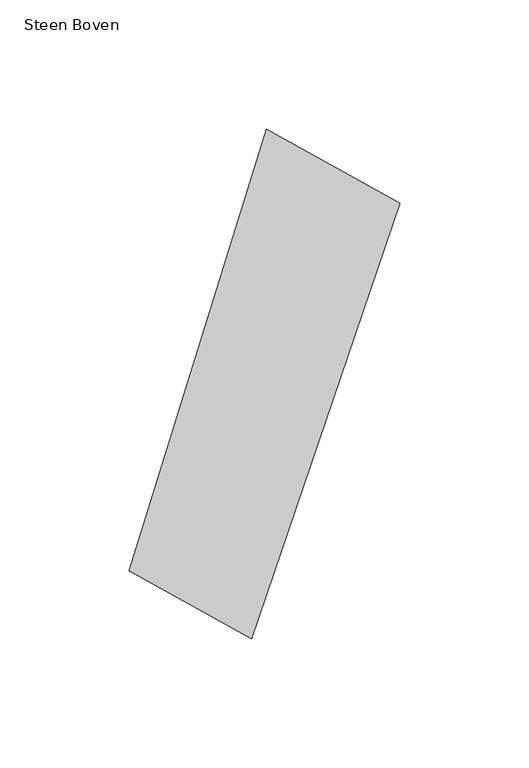
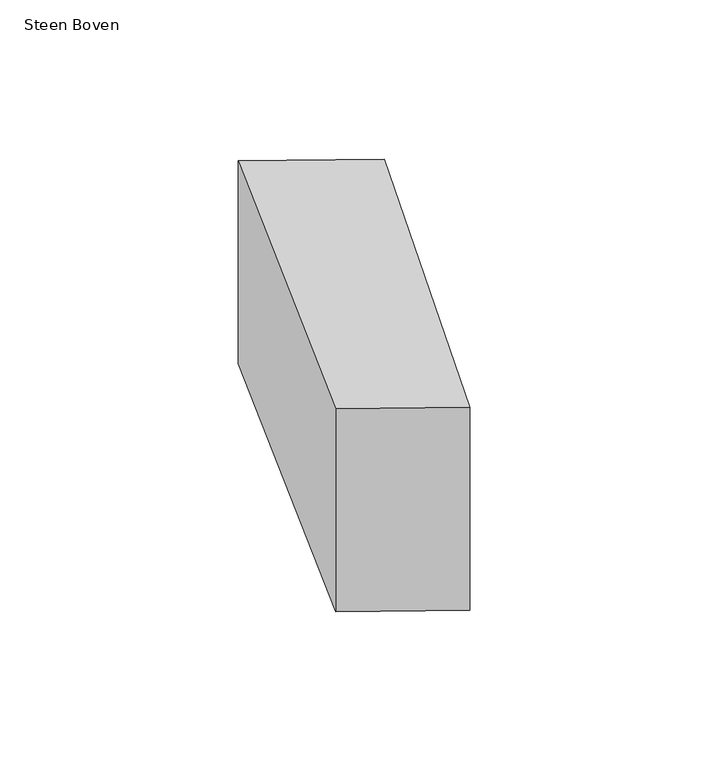
"""IFC4 building model written with IfcOpenShell, lengths in millimetres: proxy geometry, 00_GMA_steen_versie_4 : Steen Boven."""

from ifc_helpers import new_model, si_unit, origin, origin_with_axes, place, context, project, spatial, polyline, outline, extrude, source, transform, mapped, element, save


def steen_boven_75a7deea(model_context):
    return source(origin(), model_context, "Body", "SweptSolid", [
        extrude(outline(polyline([(130.6627924, 157.5699855), (73.3066538, -10.801582), (25.9422166, 15.4038976), (79.0789695, 186.1364244), (130.6627924, 157.5699855)])), origin_with_axes(), (0.0, 0.0, 1.0), 100.0),
    ])


if __name__ == "__main__":
    model = new_model("IFC4")
    model_context = context("Model", 3, world=origin())
    ifc_project = project(units=[si_unit("LENGTHUNIT", "METRE", prefix="MILLI")], contexts=[model_context])
    site = spatial("IfcSite", under=ifc_project)
    building = spatial("IfcBuilding", under=site)
    placement = place(None, origin())
    steen_boven_shape = steen_boven_75a7deea(model_context)
    element("IfcBuildingElementProxy", 1, Name="00_GMA_steen_versie_4 : Steen Boven", ObjectType="00_GMA_steen_versie_4 : Steen Boven", at=placement, inside=building, context=model_context, shape_type="MappedRepresentation", body=[
        mapped(steen_boven_shape, transform((0.0, 0.0, 0.0), x_axis=(1.0, 0.0, 0.0), y_axis=(0.0, 1.0, 0.0), z_axis=(0.0, 0.0, 1.0))),
    ])
    save(model, "model.ifc")

# Revit data of these elements
# Type "00_GMA_steen_versie_4 : Steen Boven"
#   StootVoegHalfBoven [instance default] = 5 mm
#   StootVoegHalf [instance default] = 5 mm
#   StootVoegBreedteOnder = 10 mm
#   StootVoegBreedteBoven = 10 mm
#   Steendikte = 100 mm
#   LintVoegOnderHalf = 5 mm
#   LintVoegOnder = 10 mm
#   LintVoegBovenHalf = 0 mm
#   LintVoegBoven = 0 mm
#   materiaal = none
#   MateriaalVoeg = none
#   Default Elevation = 0
